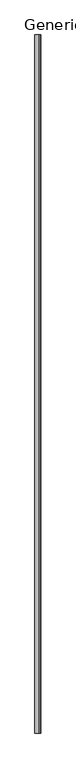
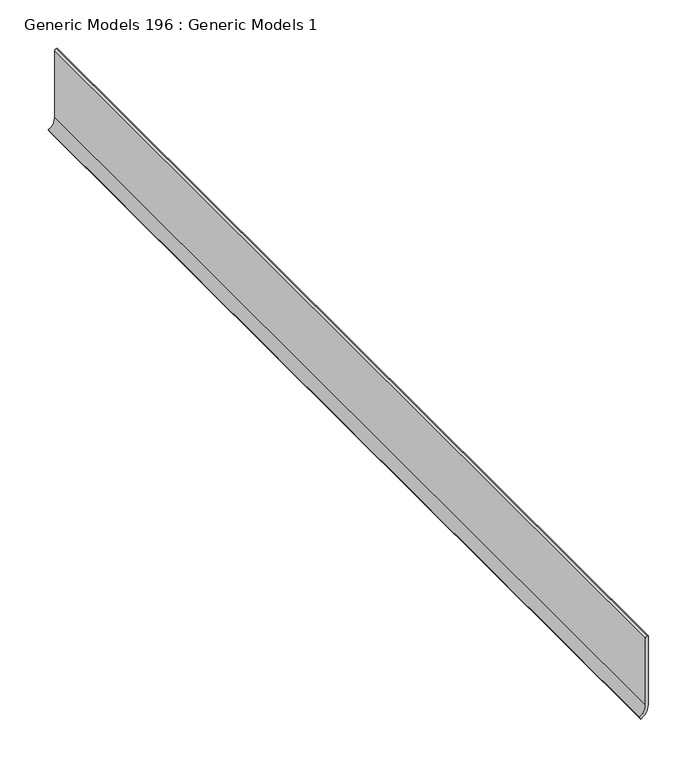
"""IFC4 building model written with IfcOpenShell, lengths in millimetres: proxy geometry, Generic Models 196 : Generic Models 1."""

import ifcopenshell
import ifcopenshell.guid

model = None  # the IFC model being written
_history = None  # IfcOwnerHistory: only IFC2X3 demands one
_inside = {}  # id of a spatial element -> (the spatial element, [elements in it])
_under = {}  # id of a project, library or spatial element -> (it, [spatial elements below it])
_declared = {}  # id of a project -> (the project, [libraries it declares])
_typed = {}  # id of a type object -> (the type object, [elements of that type])
_made_of = {}  # id of a material, layer set ... -> (it, [elements and type objects made of it])


def new_model(schema):
    """Start an empty IFC model of exactly this schema.

    Asked for "IFC4X3", IfcOpenShell would pick the latest addendum, in which some entities
    have other attributes; the version numbers below select the first issue.
    IFC2X3 requires an IfcOwnerHistory on every rooted entity: one is made here for all.
    """
    global model, _history
    if schema == "IFC4X3":
        model = ifcopenshell.file(schema_version=(4, 3, 0, 0))
    else:
        model = ifcopenshell.file(schema=schema)
    _inside.clear()
    _under.clear()
    _declared.clear()
    _typed.clear()
    _made_of.clear()
    _history = None
    if model.schema == "IFC2X3":
        org = make("IfcOrganization", Name="unknown")
        user = make(
            "IfcPersonAndOrganization",
            ThePerson=make("IfcPerson", FamilyName="unknown"),
            TheOrganization=org,
        )
        app = make(
            "IfcApplication",
            ApplicationDeveloper=org,
            Version="unknown",
            ApplicationFullName="unknown",
            ApplicationIdentifier="unknown",
        )
        _history = make(
            "IfcOwnerHistory",
            OwningUser=user,
            OwningApplication=app,
            ChangeAction="ADDED",
            CreationDate=0,
        )
    return model


def make(cls, **values):
    """One entity of the class cls with the attributes given. An attribute that is None is left unset."""
    return model.create_entity(
        cls, **{name: value for name, value in values.items() if value is not None}
    )


def rooted(cls, **values):
    """An entity with a GlobalId (a new one), such as an element, a storey or a relation."""
    return make(cls, GlobalId=ifcopenshell.guid.new(), OwnerHistory=_history, **values)


def si_unit(unit_type, name, prefix=None):
    """IfcSIUnit, for example si_unit("LENGTHUNIT", "METRE", prefix="MILLI")."""
    return make("IfcSIUnit", UnitType=unit_type, Prefix=prefix, Name=name)


def assignment(units):
    """IfcUnitAssignment: the units of a project."""
    return None if units is None else make("IfcUnitAssignment", Units=units)


def point(xyz):
    """IfcCartesianPoint."""
    return None if xyz is None else make("IfcCartesianPoint", Coordinates=xyz)


def direction(xyz):
    """IfcDirection."""
    return None if xyz is None else make("IfcDirection", DirectionRatios=xyz)


def frame(location, z_axis=None, x_axis=None):
    """IfcAxis2Placement3D, a coordinate frame: its origin and axes. An axis left out is left unset."""
    return make(
        "IfcAxis2Placement3D",
        Location=point(location),
        Axis=direction(z_axis),
        RefDirection=direction(x_axis),
    )


def frame_2d(location, x_axis=None):
    """IfcAxis2Placement2D, a coordinate frame in the plane: its origin and x axis."""
    return make(
        "IfcAxis2Placement2D", Location=point(location), RefDirection=direction(x_axis)
    )


def origin():
    """The frame at (0, 0, 0) with its axes left unset."""
    return frame((0.0, 0.0, 0.0))


def place(relative_to, where):
    """IfcLocalPlacement: puts the frame where relative to a parent placement (None: the world)."""
    return make(
        "IfcLocalPlacement", PlacementRelTo=relative_to, RelativePlacement=where
    )


def context(
    kind, dimensions, precision=None, world=None, true_north=None, identifier=None
):
    """IfcGeometricRepresentationContext, for example the 3D "Model" context."""
    return make(
        "IfcGeometricRepresentationContext",
        ContextIdentifier=identifier,
        ContextType=kind,
        CoordinateSpaceDimension=dimensions,
        Precision=precision,
        WorldCoordinateSystem=world,
        TrueNorth=true_north,
    )


def project(units=None, contexts=None):
    """IfcProject with its units and contexts."""
    return rooted(
        "IfcProject",
        Name="project",
        RepresentationContexts=contexts,
        UnitsInContext=assignment(units),
    )


def spatial(cls, under=None, at=None, **own):
    """A site, building, storey or space (cls), placed at a placement, below another one or the project."""
    s = rooted(cls, ObjectPlacement=at, **own)
    if under is not None:
        _under.setdefault(under.id(), (under, []))[1].append(s)
    return s


def polyline(points):
    """IfcPolyline through the points."""
    return make("IfcPolyline", Points=[point(p) for p in points])


def circle_curve(where, radius):
    """IfcCircle in the frame where."""
    return make("IfcCircle", Position=where, Radius=radius)


def trimmed(basis, trim1, trim2, sense, master):
    """IfcTrimmedCurve: the piece of a basis curve between two trims."""
    return make(
        "IfcTrimmedCurve",
        BasisCurve=basis,
        Trim1=trim1,
        Trim2=trim2,
        SenseAgreement=sense,
        MasterRepresentation=master,
    )


def segment(curve, same_sense, transition):
    """IfcCompositeCurveSegment."""
    return make(
        "IfcCompositeCurveSegment",
        Transition=transition,
        SameSense=same_sense,
        ParentCurve=curve,
    )


def composite_curve(segments, self_intersect=None):
    """IfcCompositeCurve: segments joined end to end."""
    return make("IfcCompositeCurve", Segments=segments, SelfIntersect=self_intersect)


def outline(outer, holes=None, kind="AREA"):
    """IfcArbitraryClosedProfileDef: a profile drawn as a closed curve; with holes, ...WithVoids."""
    if holes is None:
        return make("IfcArbitraryClosedProfileDef", ProfileType=kind, OuterCurve=outer)
    return make(
        "IfcArbitraryProfileDefWithVoids",
        ProfileType=kind,
        OuterCurve=outer,
        InnerCurves=holes,
    )


def extrude(swept, where, along, depth):
    """IfcExtrudedAreaSolid: the profile swept, set in the frame where, extruded along a direction by depth."""
    return make(
        "IfcExtrudedAreaSolid",
        SweptArea=swept,
        Position=where,
        ExtrudedDirection=direction(along),
        Depth=depth,
    )


def shape(context_of_items, identifier, shape_type, items):
    """IfcShapeRepresentation: the items that make up one representation, for example the "Body"."""
    return make(
        "IfcShapeRepresentation",
        ContextOfItems=context_of_items,
        RepresentationIdentifier=identifier,
        RepresentationType=shape_type,
        Items=items,
    )


def source(mapping_origin, context_of_items, identifier, shape_type, items):
    """IfcRepresentationMap: a shape defined once, which mapped items show again and again."""
    return make(
        "IfcRepresentationMap",
        MappingOrigin=mapping_origin,
        MappedRepresentation=shape(context_of_items, identifier, shape_type, items),
    )


def transform(
    local_origin,
    x_axis=None,
    y_axis=None,
    z_axis=None,
    scale=None,
    scale2=None,
    scale3=None,
    uniform=True,
):
    """IfcCartesianTransformationOperator3D, or its non-uniform kind. x_axis, y_axis, z_axis: its Axis1, 2, 3."""
    if uniform:
        return make(
            "IfcCartesianTransformationOperator3D",
            Axis1=direction(x_axis),
            Axis2=direction(y_axis),
            LocalOrigin=point(local_origin),
            Scale=scale,
            Axis3=direction(z_axis),
        )
    return make(
        "IfcCartesianTransformationOperator3DnonUniform",
        Axis1=direction(x_axis),
        Axis2=direction(y_axis),
        LocalOrigin=point(local_origin),
        Scale=scale,
        Axis3=direction(z_axis),
        Scale2=scale2,
        Scale3=scale3,
    )


def mapped(mapping_source, mapping_target):
    """IfcMappedItem: shows the shape of a source again, moved by a transform."""
    return make(
        "IfcMappedItem", MappingSource=mapping_source, MappingTarget=mapping_target
    )


def made_of(thing, what):
    """Note that an element or type object is made of a material, layer set ...; save() writes the relation."""
    if what is not None:
        _made_of.setdefault(what.id(), (what, []))[1].append(thing)
    return thing


def element(
    cls,
    number,
    at=None,
    inside=None,
    cuts=None,
    type_object=None,
    material=None,
    context=None,
    identifier="Body",
    shape_type=None,
    held_by="IfcProductDefinitionShape",
    body=None,
    shapes=None,
    **own,
):
    """One element of the class cls, such as IfcWall. Its Tag is "e" and its number.

    at: its placement. inside: the storey or other place that contains it. cuts: it is an
    opening in that element (IfcRelVoidsElement). A single representation is given by context,
    identifier, shape_type and body (its items); several are given by shapes. held_by: the class
    of the entity that holds the representations. save() writes the other relations.
    """
    e = rooted(cls, Tag="e%d" % number, ObjectPlacement=at, **own)
    if body is not None:
        shapes = [shape(context, identifier, shape_type, body)]
    if shapes is not None:
        e.Representation = make(held_by, Representations=shapes)
    if inside is not None:
        _inside.setdefault(inside.id(), (inside, []))[1].append(e)
    if cuts is not None:
        rooted(
            "IfcRelVoidsElement", RelatingBuildingElement=cuts, RelatedOpeningElement=e
        )
    if type_object is not None:
        _typed.setdefault(type_object.id(), (type_object, []))[1].append(e)
    return made_of(e, material)


def aggregate(whole, parts):
    """IfcRelAggregates: a whole, such as a stair, and the parts it consists of."""
    return rooted("IfcRelAggregates", RelatingObject=whole, RelatedObjects=parts)


def save(model, path):
    """Write the relations noted so far, then the file.

    IfcRelAggregates (storeys below a building ...), IfcRelContainedInSpatialStructure (elements
    in a storey), IfcRelDefinesByType, IfcRelAssociatesMaterial and IfcRelDeclares: one each for
    every whole, place, type object, material and project.
    """
    for whole, parts in _under.values():
        aggregate(whole, parts)
    for where, things in _inside.values():
        rooted(
            "IfcRelContainedInSpatialStructure",
            RelatedElements=things,
            RelatingStructure=where,
        )
    for kind, things in _typed.values():
        rooted("IfcRelDefinesByType", RelatedObjects=things, RelatingType=kind)
    for what, things in _made_of.values():
        rooted("IfcRelAssociatesMaterial", RelatedObjects=things, RelatingMaterial=what)
    for by, libraries in _declared.values():
        rooted("IfcRelDeclares", RelatingContext=by, RelatedDefinitions=libraries)
    model.write(path)


def generic_models_196_generic_models_1_c5b7b2a8(model_context):
    return source(origin(), model_context, "Body", "SweptSolid", [
        extrude(outline(composite_curve([segment(polyline([(101.6, 49676.05), (101.6, 49674.9618018)]), True, "CONTINUOUS"), segment(trimmed(circle_curve(frame_2d((99.5131982, 49674.9618018)), 2.0868018), [point((101.6, 49674.9618018))], [point((99.5131982, 49672.875))], False, "CARTESIAN"), True, "CONTINUOUS"), segment(polyline([(99.5131982, 49672.875), (15.4496307, 49672.875)]), True, "CONTINUOUS"), segment(trimmed(circle_curve(frame_2d((15.4496307, 49658.2103032)), 14.6646968), [point((15.4496307, 49672.875))], [point((2.7496307, 49665.5426516))], True, "CARTESIAN"), True, "CONTINUOUS"), segment(polyline([(2.7496307, 49665.5426516), (0.0, 49667.1301516)]), True, "CONTINUOUS"), segment(trimmed(circle_curve(frame_2d((15.4496307, 49658.2103032)), 17.8396968), [point((0.0, 49667.1301516))], [point((15.4496307, 49676.05))], False, "CARTESIAN"), True, "CONTINUOUS"), segment(polyline([(15.4496307, 49676.05), (101.6, 49676.05)]), True, "CONTINUOUS")], self_intersect=False)), frame((0.0, 0.0, 0.0), z_axis=(0.0, 1.0, 0.0), x_axis=(0.0, 0.0, 1.0)), (0.0, 0.0, 1.0), 1219.2),
    ])


if __name__ == "__main__":
    model = new_model("IFC4")
    model_context = context("Model", 3, world=origin())
    ifc_project = project(units=[si_unit("LENGTHUNIT", "METRE", prefix="MILLI")], contexts=[model_context])
    site = spatial("IfcSite", under=ifc_project)
    building = spatial("IfcBuilding", under=site)
    placement = place(None, origin())
    generic_models_196_generic_models_1_shape = generic_models_196_generic_models_1_c5b7b2a8(model_context)
    element("IfcBuildingElementProxy", 1, Name="Generic Models 196 : Generic Models 1", ObjectType="Generic Models 196 : Generic Models 1", at=placement, inside=building, context=model_context, shape_type="MappedRepresentation", body=[
        mapped(generic_models_196_generic_models_1_shape, transform((0.0, 0.0, 0.0), x_axis=(1.0, 0.0, 0.0), y_axis=(0.0, 1.0, 0.0), z_axis=(0.0, 0.0, 1.0))),
    ])
    save(model, "model.ifc")

# Revit data of these elements
# Element 1 (IfcBuildingElementProxy, "Generic Models 196 : Generic Models 1")
#   Materials on its faces: "MATCH EXISTING BASE"
# Materials
#   "MATCH EXISTING BASE": class "Generic", colour RGB 120 120 120, transparency 0, Cost = 0
